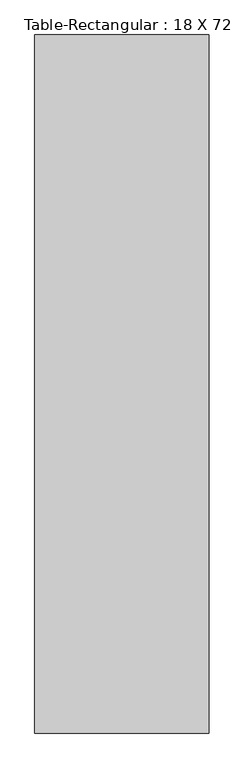
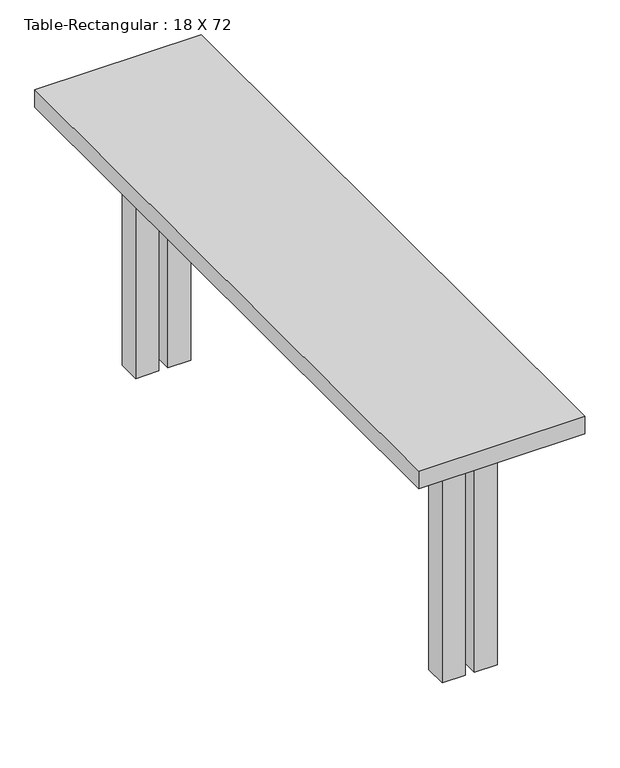
"""IFC4 building model written with IfcOpenShell, lengths in millimetres: furniture geometry, Table-Rectangular : 18 X 72."""

from ifc_helpers import new_model, si_unit, frame, origin, origin_with_axes, place, context, project, spatial, polyline, outline, extrude, source, transform, mapped, element, save


def table_rectangular_18_x_72_db6a0320(model_context):
    return source(origin(), model_context, "Body", "SweptSolid", [
        extrude(outline(polyline([(12.7, 723.9), (12.7, 698.5), (-12.7, 698.5), (-12.7, 723.9), (12.7, 723.9)])), frame((0.0, 0.0, 609.6), z_axis=(0.0, 0.0, 1.0), x_axis=(1.0, 0.0, 0.0)), (0.0, 0.0, 1.0), 101.6),
        extrude(outline(polyline([(12.7, -723.9), (-12.7, -723.9), (-12.7, -698.5), (12.7, -698.5), (12.7, -723.9)])), frame((0.0, 0.0, 609.6), z_axis=(0.0, 0.0, 1.0), x_axis=(1.0, 0.0, 0.0)), (0.0, 0.0, 1.0), 101.6),
        extrude(outline(polyline([(-25.4, -698.5), (-50.8, -698.5), (-50.8, 698.5), (-25.4, 698.5), (-25.4, -698.5)])), frame((0.0, 0.0, 609.6), z_axis=(0.0, 0.0, 1.0), x_axis=(1.0, 0.0, 0.0)), (0.0, 0.0, 1.0), 101.6),
        extrude(outline(polyline([(25.4, -698.5), (25.4, 698.5), (50.8, 698.5), (50.8, -698.5), (25.4, -698.5)])), frame((0.0, 0.0, 609.6), z_axis=(0.0, 0.0, 1.0), x_axis=(1.0, 0.0, 0.0)), (0.0, 0.0, 1.0), 101.6),
        extrude(outline(polyline([(228.6, 914.4), (228.6, -914.4), (-228.6, -914.4), (-228.6, 914.4), (228.6, 914.4)])), frame((0.0, 0.0, 711.2), z_axis=(0.0, 0.0, 1.0), x_axis=(1.0, 0.0, 0.0)), (0.0, 0.0, 1.0), 50.8),
        extrude(outline(polyline([(-12.7, 762.0), (-12.7, 698.5), (-76.2, 698.5), (-76.2, 762.0), (-12.7, 762.0)])), origin_with_axes(), (0.0, 0.0, 1.0), 711.2),
        extrude(outline(polyline([(12.7, 762.0), (76.2, 762.0), (76.2, 698.5), (12.7, 698.5), (12.7, 762.0)])), origin_with_axes(), (0.0, 0.0, 1.0), 711.2),
        extrude(outline(polyline([(-12.7, -762.0), (-76.2, -762.0), (-76.2, -698.5), (-12.7, -698.5), (-12.7, -762.0)])), origin_with_axes(), (0.0, 0.0, 1.0), 711.2),
        extrude(outline(polyline([(12.7, -762.0), (12.7, -698.5), (76.2, -698.5), (76.2, -762.0), (12.7, -762.0)])), origin_with_axes(), (0.0, 0.0, 1.0), 711.2),
    ])


if __name__ == "__main__":
    model = new_model("IFC4")
    model_context = context("Model", 3, world=origin())
    ifc_project = project(units=[si_unit("LENGTHUNIT", "METRE", prefix="MILLI")], contexts=[model_context])
    site = spatial("IfcSite", under=ifc_project)
    building = spatial("IfcBuilding", under=site)
    placement = place(None, origin())
    table_rectangular_18_x_72_shape = table_rectangular_18_x_72_db6a0320(model_context)
    element("IfcFurniture", 1, ObjectType="Table-Rectangular : 18 X 72", at=placement, inside=building, context=model_context, shape_type="MappedRepresentation", body=[
        mapped(table_rectangular_18_x_72_shape, transform((0.0, 0.0, 0.0), x_axis=(1.0, 0.0, 0.0), y_axis=(0.0, 1.0, 0.0), z_axis=(0.0, 0.0, 1.0))),
    ])
    save(model, "model.ifc")

# Revit data of these elements
# Type "Table-Rectangular : 18 X 72"
#   Assembly Code = "E2020200"
#   Height = 2' - 6"
#   Length = 1' - 6"
#   Width = 6' - 0"
#   Base Material = Wood - Birch
#   Top Material = Wood - Birch
#   Default Elevation = 0
# Element 1 (IfcFurniture, "Table-Rectangular : 18 X 72")
#   Materials on its faces: "Wood - Birch"
# Materials
#   "Wood - Birch": class "Unassigned", colour RGB 224 178 126, transparency 0
